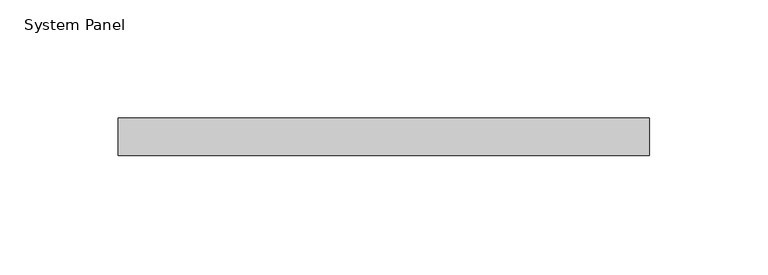
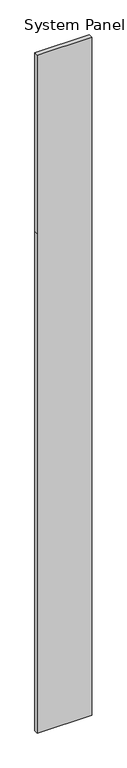
"""IFC4 building model written with IfcOpenShell, lengths in millimetres: plate geometry, System Panel : 로이복층유리_16."""

from ifc_helpers import new_model, si_unit, frame, origin, place, context, project, spatial, polyline, outline, extrude, source, transform, mapped, element, save


def system_panel_827ed390(model_context):
    return source(origin(), model_context, "Body", "SweptSolid", [
        extrude(outline(polyline([(0.0, -112.5), (0.0, 112.5), (2177.5, 112.5), (2955.0, 112.5), (2955.0, -112.5), (2177.5, -112.5), (0.0, -112.5)])), frame((0.0, -8.0, 0.0), z_axis=(0.0, 1.0, 0.0), x_axis=(0.0, 0.0, 1.0)), (0.0, 0.0, 1.0), 16.0),
    ])


if __name__ == "__main__":
    model = new_model("IFC4")
    model_context = context("Model", 3, world=origin())
    ifc_project = project(units=[si_unit("LENGTHUNIT", "METRE", prefix="MILLI")], contexts=[model_context])
    site = spatial("IfcSite", under=ifc_project)
    building = spatial("IfcBuilding", under=site)
    placement = place(None, origin())
    system_panel_shape = system_panel_827ed390(model_context)
    element("IfcPlate", 1, ObjectType="System Panel : 로이복층유리_16", at=placement, inside=building, context=model_context, shape_type="MappedRepresentation", body=[
        mapped(system_panel_shape, transform((0.0, 0.0, 0.0), x_axis=(1.0, 0.0, 0.0), y_axis=(0.0, 1.0, 0.0), z_axis=(0.0, 0.0, 1.0))),
    ])
    save(model, "model.ifc")

# Revit data of these elements
# Element 1 (IfcPlate, "System Panel : 로이복층유리_16")
#   Materials on its faces: "00_Glass_Glass"
# Materials
#   "00_Glass_Glass": class "Glass", colour RGB 218 227 224, transparency 0.85, Description = "Glass", Cost = 0, Image = none
